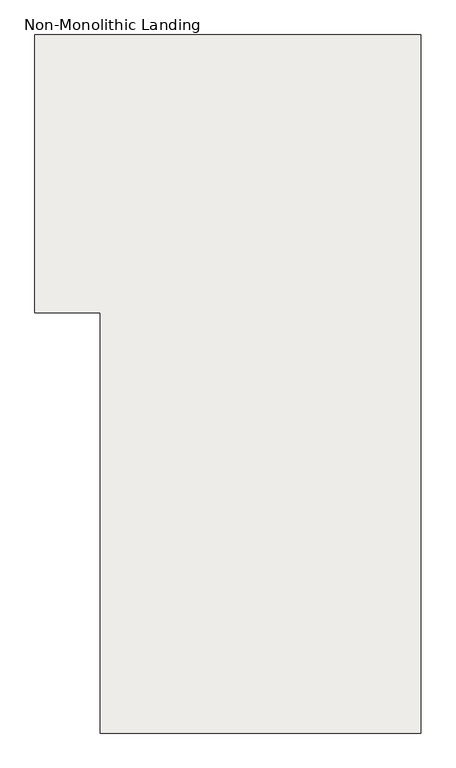
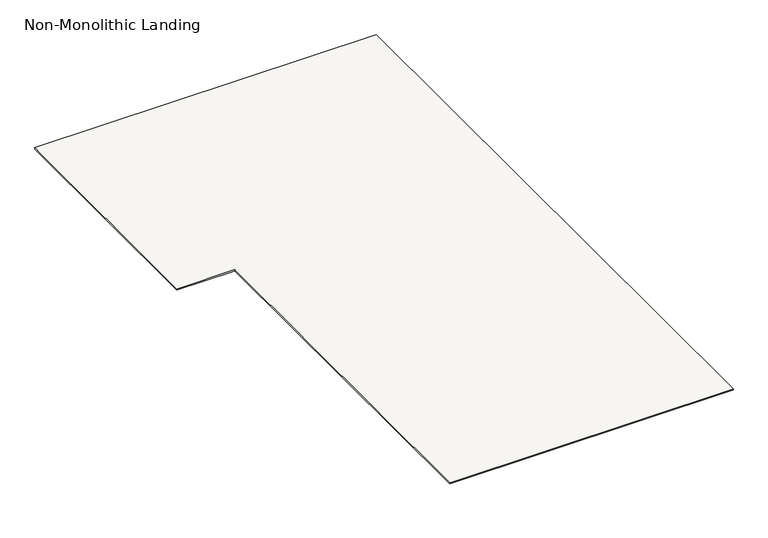
"""IFC4 building model written with IfcOpenShell, lengths in millimetres: slab geometry, Non-Monolithic Landing."""

import ifcopenshell
import ifcopenshell.guid

model = None  # the IFC model being written
_history = None  # IfcOwnerHistory: only IFC2X3 demands one
_inside = {}  # id of a spatial element -> (the spatial element, [elements in it])
_under = {}  # id of a project, library or spatial element -> (it, [spatial elements below it])
_declared = {}  # id of a project -> (the project, [libraries it declares])
_typed = {}  # id of a type object -> (the type object, [elements of that type])
_made_of = {}  # id of a material, layer set ... -> (it, [elements and type objects made of it])


def new_model(schema):
    """Start an empty IFC model of exactly this schema.

    Asked for "IFC4X3", IfcOpenShell would pick the latest addendum, in which some entities
    have other attributes; the version numbers below select the first issue.
    IFC2X3 requires an IfcOwnerHistory on every rooted entity: one is made here for all.
    """
    global model, _history
    if schema == "IFC4X3":
        model = ifcopenshell.file(schema_version=(4, 3, 0, 0))
    else:
        model = ifcopenshell.file(schema=schema)
    _inside.clear()
    _under.clear()
    _declared.clear()
    _typed.clear()
    _made_of.clear()
    _history = None
    if model.schema == "IFC2X3":
        org = make("IfcOrganization", Name="unknown")
        user = make(
            "IfcPersonAndOrganization",
            ThePerson=make("IfcPerson", FamilyName="unknown"),
            TheOrganization=org,
        )
        app = make(
            "IfcApplication",
            ApplicationDeveloper=org,
            Version="unknown",
            ApplicationFullName="unknown",
            ApplicationIdentifier="unknown",
        )
        _history = make(
            "IfcOwnerHistory",
            OwningUser=user,
            OwningApplication=app,
            ChangeAction="ADDED",
            CreationDate=0,
        )
    return model


def make(cls, **values):
    """One entity of the class cls with the attributes given. An attribute that is None is left unset."""
    return model.create_entity(
        cls, **{name: value for name, value in values.items() if value is not None}
    )


def rooted(cls, **values):
    """An entity with a GlobalId (a new one), such as an element, a storey or a relation."""
    return make(cls, GlobalId=ifcopenshell.guid.new(), OwnerHistory=_history, **values)


def si_unit(unit_type, name, prefix=None):
    """IfcSIUnit, for example si_unit("LENGTHUNIT", "METRE", prefix="MILLI")."""
    return make("IfcSIUnit", UnitType=unit_type, Prefix=prefix, Name=name)


def assignment(units):
    """IfcUnitAssignment: the units of a project."""
    return None if units is None else make("IfcUnitAssignment", Units=units)


def point(xyz):
    """IfcCartesianPoint."""
    return None if xyz is None else make("IfcCartesianPoint", Coordinates=xyz)


def direction(xyz):
    """IfcDirection."""
    return None if xyz is None else make("IfcDirection", DirectionRatios=xyz)


def frame(location, z_axis=None, x_axis=None):
    """IfcAxis2Placement3D, a coordinate frame: its origin and axes. An axis left out is left unset."""
    return make(
        "IfcAxis2Placement3D",
        Location=point(location),
        Axis=direction(z_axis),
        RefDirection=direction(x_axis),
    )


def origin():
    """The frame at (0, 0, 0) with its axes left unset."""
    return frame((0.0, 0.0, 0.0))


def place(relative_to, where):
    """IfcLocalPlacement: puts the frame where relative to a parent placement (None: the world)."""
    return make(
        "IfcLocalPlacement", PlacementRelTo=relative_to, RelativePlacement=where
    )


def context(
    kind, dimensions, precision=None, world=None, true_north=None, identifier=None
):
    """IfcGeometricRepresentationContext, for example the 3D "Model" context."""
    return make(
        "IfcGeometricRepresentationContext",
        ContextIdentifier=identifier,
        ContextType=kind,
        CoordinateSpaceDimension=dimensions,
        Precision=precision,
        WorldCoordinateSystem=world,
        TrueNorth=true_north,
    )


def project(units=None, contexts=None):
    """IfcProject with its units and contexts."""
    return rooted(
        "IfcProject",
        Name="project",
        RepresentationContexts=contexts,
        UnitsInContext=assignment(units),
    )


def spatial(cls, under=None, at=None, **own):
    """A site, building, storey or space (cls), placed at a placement, below another one or the project."""
    s = rooted(cls, ObjectPlacement=at, **own)
    if under is not None:
        _under.setdefault(under.id(), (under, []))[1].append(s)
    return s


def polyline(points):
    """IfcPolyline through the points."""
    return make("IfcPolyline", Points=[point(p) for p in points])


def outline(outer, holes=None, kind="AREA"):
    """IfcArbitraryClosedProfileDef: a profile drawn as a closed curve; with holes, ...WithVoids."""
    if holes is None:
        return make("IfcArbitraryClosedProfileDef", ProfileType=kind, OuterCurve=outer)
    return make(
        "IfcArbitraryProfileDefWithVoids",
        ProfileType=kind,
        OuterCurve=outer,
        InnerCurves=holes,
    )


def extrude(swept, where, along, depth):
    """IfcExtrudedAreaSolid: the profile swept, set in the frame where, extruded along a direction by depth."""
    return make(
        "IfcExtrudedAreaSolid",
        SweptArea=swept,
        Position=where,
        ExtrudedDirection=direction(along),
        Depth=depth,
    )


def shape(context_of_items, identifier, shape_type, items):
    """IfcShapeRepresentation: the items that make up one representation, for example the "Body"."""
    return make(
        "IfcShapeRepresentation",
        ContextOfItems=context_of_items,
        RepresentationIdentifier=identifier,
        RepresentationType=shape_type,
        Items=items,
    )


def source(mapping_origin, context_of_items, identifier, shape_type, items):
    """IfcRepresentationMap: a shape defined once, which mapped items show again and again."""
    return make(
        "IfcRepresentationMap",
        MappingOrigin=mapping_origin,
        MappedRepresentation=shape(context_of_items, identifier, shape_type, items),
    )


def transform(
    local_origin,
    x_axis=None,
    y_axis=None,
    z_axis=None,
    scale=None,
    scale2=None,
    scale3=None,
    uniform=True,
):
    """IfcCartesianTransformationOperator3D, or its non-uniform kind. x_axis, y_axis, z_axis: its Axis1, 2, 3."""
    if uniform:
        return make(
            "IfcCartesianTransformationOperator3D",
            Axis1=direction(x_axis),
            Axis2=direction(y_axis),
            LocalOrigin=point(local_origin),
            Scale=scale,
            Axis3=direction(z_axis),
        )
    return make(
        "IfcCartesianTransformationOperator3DnonUniform",
        Axis1=direction(x_axis),
        Axis2=direction(y_axis),
        LocalOrigin=point(local_origin),
        Scale=scale,
        Axis3=direction(z_axis),
        Scale2=scale2,
        Scale3=scale3,
    )


def mapped(mapping_source, mapping_target):
    """IfcMappedItem: shows the shape of a source again, moved by a transform."""
    return make(
        "IfcMappedItem", MappingSource=mapping_source, MappingTarget=mapping_target
    )


def made_of(thing, what):
    """Note that an element or type object is made of a material, layer set ...; save() writes the relation."""
    if what is not None:
        _made_of.setdefault(what.id(), (what, []))[1].append(thing)
    return thing


def element(
    cls,
    number,
    at=None,
    inside=None,
    cuts=None,
    type_object=None,
    material=None,
    context=None,
    identifier="Body",
    shape_type=None,
    held_by="IfcProductDefinitionShape",
    body=None,
    shapes=None,
    **own,
):
    """One element of the class cls, such as IfcWall. Its Tag is "e" and its number.

    at: its placement. inside: the storey or other place that contains it. cuts: it is an
    opening in that element (IfcRelVoidsElement). A single representation is given by context,
    identifier, shape_type and body (its items); several are given by shapes. held_by: the class
    of the entity that holds the representations. save() writes the other relations.
    """
    e = rooted(cls, Tag="e%d" % number, ObjectPlacement=at, **own)
    if body is not None:
        shapes = [shape(context, identifier, shape_type, body)]
    if shapes is not None:
        e.Representation = make(held_by, Representations=shapes)
    if inside is not None:
        _inside.setdefault(inside.id(), (inside, []))[1].append(e)
    if cuts is not None:
        rooted(
            "IfcRelVoidsElement", RelatingBuildingElement=cuts, RelatedOpeningElement=e
        )
    if type_object is not None:
        _typed.setdefault(type_object.id(), (type_object, []))[1].append(e)
    return made_of(e, material)


def aggregate(whole, parts):
    """IfcRelAggregates: a whole, such as a stair, and the parts it consists of."""
    return rooted("IfcRelAggregates", RelatingObject=whole, RelatedObjects=parts)


def save(model, path):
    """Write the relations noted so far, then the file.

    IfcRelAggregates (storeys below a building ...), IfcRelContainedInSpatialStructure (elements
    in a storey), IfcRelDefinesByType, IfcRelAssociatesMaterial and IfcRelDeclares: one each for
    every whole, place, type object, material and project.
    """
    for whole, parts in _under.values():
        aggregate(whole, parts)
    for where, things in _inside.values():
        rooted(
            "IfcRelContainedInSpatialStructure",
            RelatedElements=things,
            RelatingStructure=where,
        )
    for kind, things in _typed.values():
        rooted("IfcRelDefinesByType", RelatedObjects=things, RelatingType=kind)
    for what, things in _made_of.values():
        rooted("IfcRelAssociatesMaterial", RelatedObjects=things, RelatingMaterial=what)
    for by, libraries in _declared.values():
        rooted("IfcRelDeclares", RelatingContext=by, RelatedDefinitions=libraries)
    model.write(path)


def non_monolithic_landing_12d89192(model_context):
    return source(origin(), model_context, "Body", "SweptSolid", [
        extrude(outline(polyline([(-12231.0, 13220.4345331), (-12231.0, 10230.4345331), (-13603.0, 10230.4345331), (-13603.0, 12030.4345331), (-13883.4671154, 12030.4345331), (-13883.4671154, 13220.4345331), (-12231.0, 13220.4345331)])), frame((0.0, 0.0, 7994.0), z_axis=(0.0, 0.0, 1.0), x_axis=(1.0, 0.0, 0.0)), (0.0, 0.0, 1.0), 6.0),
    ])


if __name__ == "__main__":
    model = new_model("IFC4")
    model_context = context("Model", 3, world=origin())
    ifc_project = project(units=[si_unit("LENGTHUNIT", "METRE", prefix="MILLI")], contexts=[model_context])
    site = spatial("IfcSite", under=ifc_project)
    building = spatial("IfcBuilding", under=site)
    placement = place(None, origin())
    non_monolithic_landing_shape = non_monolithic_landing_12d89192(model_context)
    element("IfcSlab", 1, ObjectType="Non-Monolithic Landing", at=placement, inside=building, context=model_context, shape_type="MappedRepresentation", body=[
        mapped(non_monolithic_landing_shape, transform((0.0, 0.0, 0.0), x_axis=(1.0, 0.0, 0.0), y_axis=(0.0, 1.0, 0.0), z_axis=(0.0, 0.0, 1.0))),
    ])
    save(model, "model.ifc")

# Revit data of these elements
# Element 1 (IfcSlab, "Non-Monolithic Landing")
#   Materials on its faces: "Steel, Paint Finish, Dark Gray"
# Materials
#   "Steel, Paint Finish, Dark Gray": class "Metal", colour RGB 89 89 89, transparency 0, Description = "Steel, paint finish, dark gray, glossy", Cost = 0
